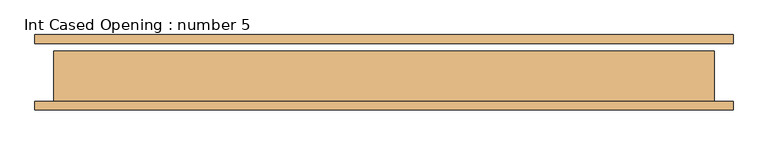
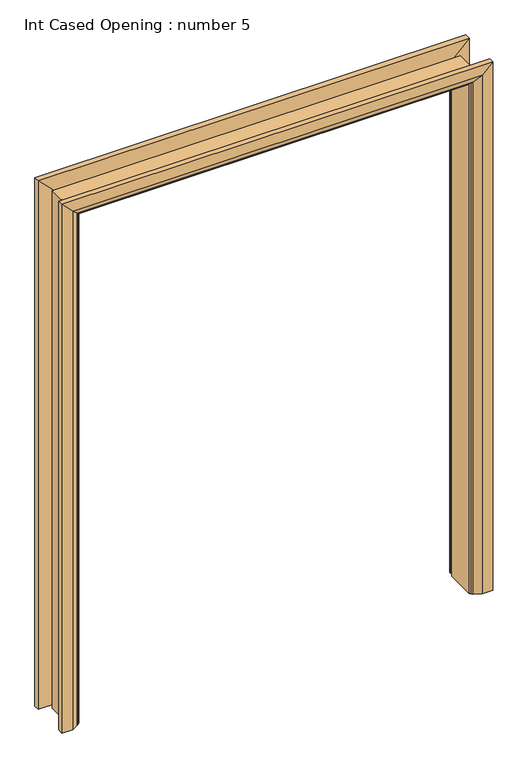
"""IFC4 building model written with IfcOpenShell, lengths in millimetres: door geometry, Int Cased Opening : number 5."""

from ifc_helpers import new_model, si_unit, frame, origin, place, context, project, spatial, circle_curve, ellipse_curve, faceted_brep, source, transform, mapped, element, save
from ifc_brep_helpers import plane_surface, cylinder_surface, advanced_brep


def int_cased_opening_number_5_fdac8540(model_context):
    return source(origin(), model_context, "Body", "SolidModel", [
        faceted_brep([(-722.0, 57.15, 0.0), (-722.0, -57.15, 0.0), (-754.0, -57.15, 0.0), (-754.0, 57.15, 0.0), (-722.0, 57.15, 1992.0), (-722.0, -57.15, 1992.0), (-754.0, -57.15, 2024.0), (-754.0, 57.15, 2024.0), (722.0, 57.15, 0.0), (754.0, 57.15, 0.0), (754.0, -57.15, 0.0), (722.0, -57.15, 0.0), (722.0, 57.15, 1992.0), (754.0, 57.15, 2024.0), (754.0, -57.15, 2024.0), (722.0, -57.15, 1992.0)], [[[0, 1, 2, 3]], [[1, 0, 4, 5]], [[2, 1, 5, 6]], [[3, 2, 6, 7]], [[0, 3, 7, 4]], [[8, 9, 10, 11]], [[12, 13, 9, 8]], [[13, 14, 10, 9]], [[14, 15, 11, 10]], [[15, 12, 8, 11]], [[5, 4, 12, 15]], [[6, 5, 15, 14]], [[7, 6, 14, 13]], [[4, 7, 13, 12]]]),
        advanced_brep(
        [(-797.0, 95.0, 0.0), (-757.0, 95.0, 0.0), (-731.0, 81.0, 0.0), (-727.0, 75.0, 0.0), (-797.0, 75.0, 0.0), (-797.0, 95.0, 2067.0), (-757.0, 95.0, 2027.0), (-731.0, 81.0, 2001.0), (-727.0, 75.0, 1997.0), (-797.0, 75.0, 2067.0), (797.0, 95.0, 2067.0), (757.0, 95.0, 2027.0), (731.0, 81.0, 2001.0), (727.0, 75.0, 1997.0), (797.0, 75.0, 2067.0), (797.0, 95.0, 0.0), (797.0, 75.0, 0.0), (727.0, 75.0, 0.0), (731.0, 81.0, 0.0), (757.0, 95.0, 0.0)],
        [
            (0, 1),
            (1, 2),
            (2, 3, circle_curve(frame((-735.0, 74.0, 0.0), z_axis=(0.0, 0.0, -1.0), x_axis=(-1.0, 0.0, 0.0)), 8.0622577)),
            (3, 4),
            (4, 0),
            (0, 5),
            (5, 6),
            (6, 1),
            (6, 7),
            (7, 2),
            (7, 8, ellipse_curve(frame((-735.0, 74.0, 2005.0), z_axis=(-0.7071067811865475, 0.0, -0.7071067811865475), x_axis=(0.7071067811865474, 0.0, -0.7071067811865476)), 11.4017543, 8.0622577)),
            (8, 3),
            (8, 9),
            (9, 4),
            (9, 5),
            (5, 10),
            (10, 11),
            (11, 6),
            (11, 12),
            (12, 7),
            (12, 13, ellipse_curve(frame((735.0, 74.0, 2005.0), z_axis=(-0.7071067811865475, 0.0, 0.7071067811865475), x_axis=(-0.7071067811865476, 0.0, -0.7071067811865474)), 11.4017543, 8.0622577)),
            (13, 8),
            (13, 14),
            (14, 9),
            (14, 10),
            (15, 16),
            (16, 17),
            (17, 18, circle_curve(frame((735.0, 74.0, 0.0), z_axis=(0.0, 0.0, -1.0), x_axis=(1.0, 0.0, 0.0)), 8.0622577)),
            (18, 19),
            (19, 15),
            (10, 15),
            (19, 11),
            (18, 12),
            (17, 13),
            (16, 14),
        ],
        [
            plane_surface(frame((-727.0, 2.1989011, 0.0), z_axis=(0.0, 0.0, -1.0), x_axis=(1.0, 0.0, 0.0))),
            plane_surface(frame((-797.0, 95.0, 0.0), z_axis=(0.0, 1.0, 0.0), x_axis=(0.0, 0.0, 1.0))),
            plane_surface(frame((-757.0, 95.0, 0.0), z_axis=(0.4740998230350183, 0.8804710999221749, 0.0), x_axis=(0.0, 0.0, 1.0))),
            cylinder_surface(frame((-735.0, 74.0, 0.0), z_axis=(0.0, 0.0, -1.0), x_axis=(-1.0, 0.0, 0.0)), 8.0622577),
            plane_surface(frame((-727.0, 75.0, 0.0), z_axis=(0.0, -1.0, 0.0), x_axis=(0.0, 0.0, 1.0))),
            plane_surface(frame((-797.0, 75.0, 0.0), z_axis=(-1.0, 0.0, 0.0), x_axis=(0.0, 0.0, 1.0))),
            plane_surface(frame((-797.0, 95.0, 2067.0), z_axis=(0.0, 1.0, 0.0), x_axis=(1.0, 0.0, 0.0))),
            plane_surface(frame((-757.0, 95.0, 2027.0), z_axis=(0.0, 0.8804710999221749, -0.4740998230350183), x_axis=(1.0, 0.0, 0.0))),
            cylinder_surface(frame((-727.0, 74.0, 2005.0), z_axis=(-1.0, 0.0, 0.0), x_axis=(0.0, 0.0, 1.0)), 8.0622577),
            plane_surface(frame((-727.0, 75.0, 1997.0), z_axis=(0.0, -1.0, 0.0), x_axis=(1.0, 0.0, 0.0))),
            plane_surface(frame((-797.0, 75.0, 2067.0), z_axis=(0.0, 0.0, 1.0), x_axis=(1.0, 0.0, 0.0))),
            plane_surface(frame((727.0, 2.1989011, 0.0), z_axis=(0.0, 0.0, -1.0), x_axis=(-1.0, 0.0, 0.0))),
            plane_surface(frame((797.0, 95.0, 2067.0), z_axis=(0.0, 1.0, 0.0), x_axis=(0.0, 0.0, -1.0))),
            plane_surface(frame((757.0, 95.0, 2027.0), z_axis=(-0.4740998230350183, 0.8804710999221749, 0.0), x_axis=(0.0, 0.0, -1.0))),
            cylinder_surface(frame((735.0, 74.0, 1997.0), z_axis=(0.0, 0.0, 1.0), x_axis=(1.0, 0.0, 0.0)), 8.0622577),
            plane_surface(frame((727.0, 75.0, 1997.0), z_axis=(0.0, -1.0, 0.0), x_axis=(0.0, 0.0, -1.0))),
            plane_surface(frame((797.0, 75.0, 2067.0), z_axis=(1.0, 0.0, 0.0), x_axis=(0.0, 0.0, -1.0))),
        ],
        [
            (0, [[1, 2, 3, 4, 5]]),
            (1, [[-1, 6, 7, 8]]),
            (2, [[-2, -8, 9, 10]]),
            (3, [[-3, -10, 11, 12]]),
            (4, [[-4, -12, 13, 14]]),
            (5, [[-5, -14, 15, -6]]),
            (6, [[-7, 16, 17, 18]]),
            (7, [[-9, -18, 19, 20]]),
            (8, [[-11, -20, 21, 22]]),
            (9, [[-13, -22, 23, 24]]),
            (10, [[-15, -24, 25, -16]]),
            (11, [[26, 27, 28, 29, 30]]),
            (12, [[-17, 31, -30, 32]]),
            (13, [[-19, -32, -29, 33]]),
            (14, [[-21, -33, -28, 34]]),
            (15, [[-23, -34, -27, 35]]),
            (16, [[-25, -35, -26, -31]]),
        ],
    ),
        advanced_brep(
        [(-797.0, -77.15, 0.0), (-797.0, -57.15, 0.0), (-727.0, -57.15, 0.0), (-731.0, -63.15, 0.0), (-757.0, -77.15, 0.0), (-797.0, -77.15, 2067.0), (-797.0, -57.15, 2067.0), (-727.0, -57.15, 1997.0), (-731.0, -63.15, 2001.0), (-757.0, -77.15, 2027.0), (797.0, -77.15, 2067.0), (797.0, -57.15, 2067.0), (727.0, -57.15, 1997.0), (731.0, -63.15, 2001.0), (757.0, -77.15, 2027.0), (797.0, -77.15, 0.0), (757.0, -77.15, 0.0), (731.0, -63.15, 0.0), (727.0, -57.15, 0.0), (797.0, -57.15, 0.0)],
        [
            (0, 1),
            (1, 2),
            (2, 3, circle_curve(frame((-735.0, -56.15, 0.0), z_axis=(0.0, 0.0, -1.0), x_axis=(-1.0, 0.0, 0.0)), 8.0622577)),
            (3, 4),
            (4, 0),
            (0, 5),
            (5, 6),
            (6, 1),
            (6, 7),
            (7, 2),
            (7, 8, ellipse_curve(frame((-735.0, -56.15, 2005.0), z_axis=(-0.7071067811865475, 0.0, -0.7071067811865475), x_axis=(0.7071067811865474, 0.0, -0.7071067811865476)), 11.4017543, 8.0622577)),
            (8, 3),
            (8, 9),
            (9, 4),
            (9, 5),
            (5, 10),
            (10, 11),
            (11, 6),
            (11, 12),
            (12, 7),
            (12, 13, ellipse_curve(frame((735.0, -56.15, 2005.0), z_axis=(-0.7071067811865475, 0.0, 0.7071067811865475), x_axis=(-0.7071067811865476, 0.0, -0.7071067811865474)), 11.4017543, 8.0622577)),
            (13, 8),
            (13, 14),
            (14, 9),
            (14, 10),
            (15, 16),
            (16, 17),
            (17, 18, circle_curve(frame((735.0, -56.15, 0.0), z_axis=(0.0, 0.0, -1.0), x_axis=(1.0, 0.0, 0.0)), 8.0622577)),
            (18, 19),
            (19, 15),
            (10, 15),
            (19, 11),
            (18, 12),
            (17, 13),
            (16, 14),
        ],
        [
            plane_surface(frame((-727.0, -129.9510989, 0.0), z_axis=(0.0, 0.0, -1.0), x_axis=(1.0, 0.0, 0.0))),
            plane_surface(frame((-797.0, -77.15, 0.0), z_axis=(-1.0, 0.0, 0.0), x_axis=(0.0, 0.0, 1.0))),
            plane_surface(frame((-797.0, -57.15, 0.0), z_axis=(0.0, 1.0, 0.0), x_axis=(0.0, 0.0, 1.0))),
            cylinder_surface(frame((-735.0, -56.15, 0.0), z_axis=(0.0, 0.0, -1.0), x_axis=(-1.0, 0.0, 0.0)), 8.0622577),
            plane_surface(frame((-731.0, -63.15, 0.0), z_axis=(0.4740998230350183, -0.8804710999221749, 0.0), x_axis=(0.0, 0.0, 1.0))),
            plane_surface(frame((-757.0, -77.15, 0.0), z_axis=(0.0, -1.0, 0.0), x_axis=(0.0, 0.0, 1.0))),
            plane_surface(frame((-797.0, -77.15, 2067.0), z_axis=(0.0, 0.0, 1.0), x_axis=(1.0, 0.0, 0.0))),
            plane_surface(frame((-797.0, -57.15, 2067.0), z_axis=(0.0, 1.0, 0.0), x_axis=(1.0, 0.0, 0.0))),
            cylinder_surface(frame((-727.0, -56.15, 2005.0), z_axis=(-1.0, 0.0, 0.0), x_axis=(0.0, 0.0, 1.0)), 8.0622577),
            plane_surface(frame((-731.0, -63.15, 2001.0), z_axis=(0.0, -0.8804710999221749, -0.4740998230350183), x_axis=(1.0, 0.0, 0.0))),
            plane_surface(frame((-757.0, -77.15, 2027.0), z_axis=(0.0, -1.0, 0.0), x_axis=(1.0, 0.0, 0.0))),
            plane_surface(frame((727.0, -129.9510989, 0.0), z_axis=(0.0, 0.0, -1.0), x_axis=(-1.0, 0.0, 0.0))),
            plane_surface(frame((797.0, -77.15, 2067.0), z_axis=(1.0, 0.0, 0.0), x_axis=(0.0, 0.0, -1.0))),
            plane_surface(frame((797.0, -57.15, 2067.0), z_axis=(0.0, 1.0, 0.0), x_axis=(0.0, 0.0, -1.0))),
            cylinder_surface(frame((735.0, -56.15, 1997.0), z_axis=(0.0, 0.0, 1.0), x_axis=(1.0, 0.0, 0.0)), 8.0622577),
            plane_surface(frame((731.0, -63.15, 2001.0), z_axis=(-0.4740998230350183, -0.8804710999221749, 0.0), x_axis=(0.0, 0.0, -1.0))),
            plane_surface(frame((757.0, -77.15, 2027.0), z_axis=(0.0, -1.0, 0.0), x_axis=(0.0, 0.0, -1.0))),
        ],
        [
            (0, [[1, 2, 3, 4, 5]]),
            (1, [[-1, 6, 7, 8]]),
            (2, [[-2, -8, 9, 10]]),
            (3, [[-3, -10, 11, 12]]),
            (4, [[-4, -12, 13, 14]]),
            (5, [[-5, -14, 15, -6]]),
            (6, [[-7, 16, 17, 18]]),
            (7, [[-9, -18, 19, 20]]),
            (8, [[-11, -20, 21, 22]]),
            (9, [[-13, -22, 23, 24]]),
            (10, [[-15, -24, 25, -16]]),
            (11, [[26, 27, 28, 29, 30]]),
            (12, [[-17, 31, -30, 32]]),
            (13, [[-19, -32, -29, 33]]),
            (14, [[-21, -33, -28, 34]]),
            (15, [[-23, -34, -27, 35]]),
            (16, [[-25, -35, -26, -31]]),
        ],
    ),
    ])


if __name__ == "__main__":
    model = new_model("IFC4")
    model_context = context("Model", 3, world=origin())
    ifc_project = project(units=[si_unit("LENGTHUNIT", "METRE", prefix="MILLI")], contexts=[model_context])
    site = spatial("IfcSite", under=ifc_project)
    building = spatial("IfcBuilding", under=site)
    placement = place(None, origin())
    int_cased_opening_number_5_shape = int_cased_opening_number_5_fdac8540(model_context)
    element("IfcDoor", 1, ObjectType="Int Cased Opening : number 5", at=placement, inside=building, context=model_context, shape_type="MappedRepresentation", body=[
        mapped(int_cased_opening_number_5_shape, transform((0.0, 0.0, 0.0), x_axis=(1.0, 0.0, 0.0), y_axis=(0.0, 1.0, 0.0), z_axis=(0.0, 0.0, 1.0))),
    ])
    save(model, "model.ifc")

# Revit data of these elements
# Type "Int Cased Opening : number 5"
#   Type Mark = "105"
#   Operation = "UserDefined"
#   Manufacturer = "Revit"
#   Keynote = "L20"
#   Width = 5' - 0"
#   Rough Width = 5' - 0"
#   Rough Height = 6' - 8"
#   Height = 6' - 8"
#   Frame Thickness = 0' - 1.25984"
#   Architrave Setback = 0' - 0.19685"
#   Vis - Architrave = yes
#   Material Frame = Door - Frame/Mullion
#   Material Architrave = Door - Architrave
#   Function = (empty or 0)
#   Wall Closure = (empty or 0)
# Element 1 (IfcDoor, "Int Cased Opening : number 5")
#   Materials on its faces: "Door - Architrave", "Door - Frame/Mullion"
# Materials
#   "Door - Frame/Mullion": class "Wood", colour RGB 212 179 113, transparency 0, Keynote = "L20", Cost = 0
#   "Door - Architrave": class "Wood", colour RGB 192 192 192, transparency 0, Keynote = "P20", Cost = 0
